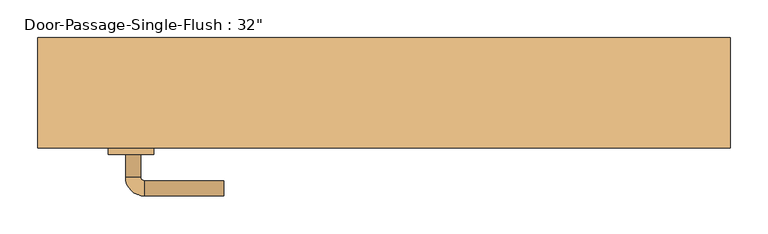
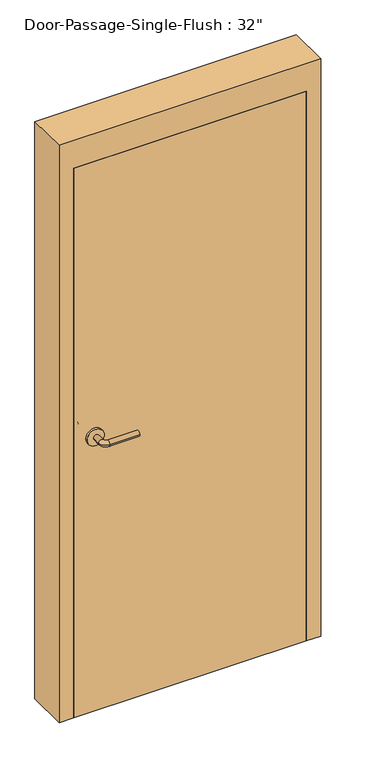
"""IFC4 building model written with IfcOpenShell, lengths in millimetres: door geometry."""

from ifc_helpers import new_model, si_unit, point, frame, frame_2d, origin, origin_with_axes, place, context, project, spatial, polyline, circle_curve, ellipse_curve, trimmed, segment, composite_curve, outline, extrude, faceted_brep, source, transform, mapped, element, save
from ifc_brep_helpers import plane_surface, cylinder_surface, revolved_surface, advanced_brep


def door_48051af7(model_context):
    return source(origin(), model_context, "Body", "SolidModel", [
        advanced_brep(
        [(-341.390625, 3.2375, 1016.0), (-321.390625, 3.2375, 1016.0), (-341.390625, 33.2375, 1016.0), (-321.390625, 33.2375, 1016.0), (-316.390625, 38.2375, 1016.0), (-316.390625, 58.2375, 1016.0), (-211.390625, 58.2375, 1016.0), (-211.390625, 38.2375, 1016.0)],
        [
            (0, 1, circle_curve(frame((-331.390625, 3.2375, 1016.0), z_axis=(0.0, -1.0, 0.0), x_axis=(1.0, 0.0, 0.0)), 10.0)),
            (1, 0, circle_curve(frame((-331.390625, 3.2375, 1016.0), z_axis=(0.0, -1.0, 0.0), x_axis=(1.0, 0.0, 0.0)), 10.0)),
            (0, 2),
            (2, 3, circle_curve(frame((-331.390625, 33.2375, 1016.0), z_axis=(0.0, -1.0, 0.0), x_axis=(1.0, 0.0, 0.0)), 10.0)),
            (3, 1),
            (3, 2, circle_curve(frame((-331.390625, 33.2375, 1016.0), z_axis=(0.0, -1.0, 0.0), x_axis=(1.0, 0.0, 0.0)), 10.0)),
            (4, 3, circle_curve(frame((-316.390625, 33.2375, 1016.0), z_axis=(0.0, 0.0, 1.0), x_axis=(-1.0, 0.0, 0.0)), 5.0)),
            (2, 5, circle_curve(frame((-316.390625, 33.2375, 1016.0), z_axis=(0.0, 0.0, -1.0), x_axis=(-1.0, 0.0, 0.0)), 25.0)),
            (5, 4, circle_curve(frame((-316.390625, 48.2375, 1016.0), z_axis=(-1.0, 0.0, 0.0), x_axis=(0.0, -1.0, 0.0)), 10.0)),
            (4, 5, circle_curve(frame((-316.390625, 48.2375, 1016.0), z_axis=(-1.0, 0.0, 0.0), x_axis=(0.0, -1.0, 0.0)), 10.0)),
            (6, 7, circle_curve(frame((-211.390625, 48.2375, 1016.0), z_axis=(1.0, 0.0, 0.0), x_axis=(0.0, -1.0, 0.0)), 10.0)),
            (7, 6, circle_curve(frame((-211.390625, 48.2375, 1016.0), z_axis=(1.0, 0.0, 0.0), x_axis=(0.0, -1.0, 0.0)), 10.0)),
            (5, 6),
            (7, 4),
        ],
        [
            plane_surface(frame((-331.390625, 3.2375, 1016.0), z_axis=(0.0, -1.0, 0.0), x_axis=(0.0, 0.0, 1.0))),
            cylinder_surface(frame((-331.390625, 3.2375, 1016.0), z_axis=(0.0, -1.0, 0.0), x_axis=(1.0, 0.0, 0.0)), 10.0),
            revolved_surface(trimmed(ellipse_curve(frame((-331.390625, 33.2375, 1016.0), z_axis=(0.0, -1.0, 0.0), x_axis=(1.0, 0.0, 0.0)), 10.0, 10.0), [point((-341.390625, 33.2375, 1016.0))], [point((-321.390625, 33.2375, 1016.0))], True, "CARTESIAN"), (-316.390625, 33.2375, 1016.0), (0.0, 0.0, -1.0)),
            revolved_surface(trimmed(ellipse_curve(frame((-331.390625, 33.2375, 1016.0), z_axis=(0.0, -1.0, 0.0), x_axis=(1.0, 0.0, 0.0)), 10.0, 10.0), [point((-321.390625, 33.2375, 1016.0))], [point((-341.390625, 33.2375, 1016.0))], True, "CARTESIAN"), (-316.390625, 33.2375, 1016.0), (0.0, 0.0, -1.0)),
            plane_surface(frame((-211.390625, 48.2375, 1016.0), z_axis=(1.0, 0.0, 0.0), x_axis=(0.0, 0.0, 1.0))),
            cylinder_surface(frame((-316.390625, 48.2375, 1016.0), z_axis=(-1.0, 0.0, 0.0), x_axis=(0.0, -1.0, 0.0)), 10.0),
        ],
        [
            (0, [[1, 2]]),
            (1, [[-1, 3, 4, 5]]),
            (1, [[-2, -5, 6, -3]]),
            (2, [[7, -4, 8, 9]]),
            (3, [[-8, -6, -7, 10]]),
            (4, [[11, 12]]),
            (5, [[-9, 13, -12, 14]]),
            (5, [[-10, -14, -11, -13]]),
        ],
    ),
        extrude(outline(composite_curve([segment(trimmed(circle_curve(frame_2d((1016.0, -333.890625)), 30.0), [point((1016.0, -363.890625))], [point((1016.0, -303.890625))], False, "CARTESIAN"), True, "CONTINUOUS"), segment(trimmed(circle_curve(frame_2d((1016.0, -333.890625)), 30.0), [point((1016.0, -303.890625))], [point((1016.0, -363.890625))], False, "CARTESIAN"), True, "CONTINUOUS")], self_intersect=False)), frame((0.0, -4.7625, 0.0), z_axis=(0.0, 1.0, 0.0), x_axis=(0.0, 0.0, 1.0)), (0.0, 0.0, 1.0), 8.0),
        advanced_brep(
        [(-341.390625, -57.2125, 1016.0), (-321.390625, -57.2125, 1016.0), (-321.390625, -87.2125, 1016.0), (-341.390625, -87.2125, 1016.0), (-316.390625, -92.2125, 1016.0), (-316.390625, -112.2125, 1016.0), (-211.390625, -112.2125, 1016.0), (-211.390625, -92.2125, 1016.0)],
        [
            (0, 1, circle_curve(frame((-331.390625, -57.2125, 1016.0), z_axis=(0.0, 1.0, 0.0), x_axis=(1.0, 0.0, 0.0)), 10.0)),
            (1, 0, circle_curve(frame((-331.390625, -57.2125, 1016.0), z_axis=(0.0, 1.0, 0.0), x_axis=(1.0, 0.0, 0.0)), 10.0)),
            (1, 2),
            (2, 3, circle_curve(frame((-331.390625, -87.2125, 1016.0), z_axis=(0.0, 1.0, 0.0), x_axis=(1.0, 0.0, 0.0)), 10.0)),
            (3, 0),
            (3, 2, circle_curve(frame((-331.390625, -87.2125, 1016.0), z_axis=(0.0, 1.0, 0.0), x_axis=(1.0, 0.0, 0.0)), 10.0)),
            (4, 5, circle_curve(frame((-316.390625, -102.2125, 1016.0), z_axis=(-1.0, 0.0, 0.0), x_axis=(0.0, 1.0, 0.0)), 10.0)),
            (5, 3, circle_curve(frame((-316.390625, -87.2125, 1016.0), z_axis=(0.0, 0.0, -1.0), x_axis=(-1.0, 0.0, 0.0)), 25.0)),
            (2, 4, circle_curve(frame((-316.390625, -87.2125, 1016.0), z_axis=(0.0, 0.0, 1.0), x_axis=(-1.0, 0.0, 0.0)), 5.0)),
            (5, 4, circle_curve(frame((-316.390625, -102.2125, 1016.0), z_axis=(-1.0, 0.0, 0.0), x_axis=(0.0, 1.0, 0.0)), 10.0)),
            (6, 7, circle_curve(frame((-211.390625, -102.2125, 1016.0), z_axis=(1.0, 0.0, 0.0), x_axis=(0.0, 1.0, 0.0)), 10.0)),
            (7, 6, circle_curve(frame((-211.390625, -102.2125, 1016.0), z_axis=(1.0, 0.0, 0.0), x_axis=(0.0, 1.0, 0.0)), 10.0)),
            (4, 7),
            (6, 5),
        ],
        [
            plane_surface(frame((-331.390625, -57.2125, 1016.0), z_axis=(0.0, 1.0, 0.0), x_axis=(0.0, 0.0, 1.0))),
            cylinder_surface(frame((-331.390625, -57.2125, 1016.0), z_axis=(0.0, 1.0, 0.0), x_axis=(1.0, 0.0, 0.0)), 10.0),
            revolved_surface(trimmed(ellipse_curve(frame((-331.390625, -87.2125, 1016.0), z_axis=(0.0, -1.0, 0.0), x_axis=(1.0, 0.0, 0.0)), 10.0, 10.0), [point((-341.390625, -87.2125, 1016.0))], [point((-321.390625, -87.2125, 1016.0))], True, "CARTESIAN"), (-316.390625, -87.2125, 1016.0), (0.0, 0.0, -1.0)),
            revolved_surface(trimmed(ellipse_curve(frame((-331.390625, -87.2125, 1016.0), z_axis=(0.0, -1.0, 0.0), x_axis=(1.0, 0.0, 0.0)), 10.0, 10.0), [point((-321.390625, -87.2125, 1016.0))], [point((-341.390625, -87.2125, 1016.0))], True, "CARTESIAN"), (-316.390625, -87.2125, 1016.0), (0.0, 0.0, -1.0)),
            plane_surface(frame((-211.390625, -102.2125, 1016.0), z_axis=(1.0, 0.0, 0.0), x_axis=(0.0, 0.0, 1.0))),
            cylinder_surface(frame((-316.390625, -102.2125, 1016.0), z_axis=(-1.0, 0.0, 0.0), x_axis=(0.0, 1.0, 0.0)), 10.0),
        ],
        [
            (0, [[1, 2]]),
            (1, [[3, 4, 5, -2]]),
            (1, [[-5, 6, -3, -1]]),
            (2, [[7, 8, -4, 9]]),
            (3, [[10, -9, -6, -8]]),
            (4, [[11, 12]]),
            (5, [[13, -11, 14, -7]]),
            (5, [[-14, -12, -13, -10]]),
        ],
    ),
        extrude(outline(composite_curve([segment(trimmed(circle_curve(frame_2d((1016.0, -333.890625)), 30.0), [point((1016.0, -363.890625))], [point((1016.0, -303.890625))], False, "CARTESIAN"), True, "CONTINUOUS"), segment(trimmed(circle_curve(frame_2d((1016.0, -333.890625)), 30.0), [point((1016.0, -303.890625))], [point((1016.0, -363.890625))], False, "CARTESIAN"), True, "CONTINUOUS")], self_intersect=False)), frame((0.0, -57.2125, 0.0), z_axis=(0.0, 1.0, 0.0), x_axis=(0.0, 0.0, 1.0)), (0.0, 0.0, 1.0), 8.0),
        faceted_brep([(406.4, 0.0, 0.0), (390.525, 0.0, 0.0), (390.525, 47.625, 0.0), (406.4, 47.625, 0.0), (406.4, 96.8375, 0.0), (457.2, 96.8375, 0.0), (457.2, -49.2125, 0.0), (406.4, -49.2125, 0.0), (406.4, -49.2125, 2032.0), (406.4, 0.0, 2032.0), (457.2, -49.2125, 2133.6), (-457.2, -49.2125, 2133.6), (-457.2, -49.2125, 0.0), (-406.4, -49.2125, 0.0), (-406.4, -49.2125, 2032.0), (457.2, 96.8375, 2133.6), (406.4, 96.8375, 2032.0), (-406.4, 96.8375, 2032.0), (-406.4, 96.8375, 0.0), (-457.2, 96.8375, 0.0), (-457.2, 96.8375, 2133.6), (406.4, 47.625, 2032.0), (390.525, 47.625, 2016.125), (-390.525, 47.625, 2016.125), (-390.525, 47.625, 0.0), (-406.4, 47.625, 0.0), (-406.4, 47.625, 2032.0), (390.525, 0.0, 2016.125), (-406.4, 0.0, 2032.0), (-406.4, 0.0, 0.0), (-390.525, 0.0, 0.0), (-390.525, 0.0, 2016.125)], [[[0, 1, 2, 3, 4, 5, 6, 7]], [[7, 8, 9, 0]], [[6, 10, 11, 12, 13, 14, 8, 7]], [[5, 15, 10, 6]], [[4, 16, 17, 18, 19, 20, 15, 5]], [[3, 21, 16, 4]], [[2, 22, 23, 24, 25, 26, 21, 3]], [[1, 27, 22, 2]], [[0, 9, 28, 29, 30, 31, 27, 1]], [[8, 14, 28, 9]], [[16, 21, 26, 17]], [[22, 27, 31, 23]], [[12, 19, 18, 25, 24, 30, 29, 13]], [[13, 29, 28, 14]], [[11, 20, 19, 12]], [[17, 26, 25, 18]], [[23, 31, 30, 24]], [[15, 20, 11, 10]]]),
        extrude(outline(polyline([(406.4, -4.7625), (406.4, -49.2125), (-406.4, -49.2125), (-406.4, -4.7625), (406.4, -4.7625)])), origin_with_axes(), (0.0, 0.0, 1.0), 2032.0),
    ])


if __name__ == "__main__":
    model = new_model("IFC4")
    model_context = context("Model", 3, world=origin())
    ifc_project = project(units=[si_unit("LENGTHUNIT", "METRE", prefix="MILLI")], contexts=[model_context])
    site = spatial("IfcSite", under=ifc_project)
    building = spatial("IfcBuilding", under=site)
    placement = place(None, origin())
    door_shape = door_48051af7(model_context)
    element("IfcDoor", 1, ObjectType="Door-Passage-Single-Flush : 32\"", at=placement, inside=building, context=model_context, shape_type="MappedRepresentation", body=[
        mapped(door_shape, transform((0.0, 0.0, 0.0), x_axis=(1.0, 0.0, 0.0), y_axis=(0.0, 1.0, 0.0), z_axis=(0.0, 0.0, 1.0))),
    ])
    save(model, "model.ifc")

# Revit data of these elements
# Type "Door-Passage-Single-Flush : 32\""
#   Type Mark = "42"
#   Assembly Code = "B2030200"
#   Analytic Construction = "Wooden"
#   Thickness = 0' - 1 3/4"
#   Thermal Resistance (R) = 0.455703 (m²·K)/W
#   Swing Angle [instance default] = 90.00°
#   Strike Height = 3' - 4"
#   Rough Width [instance default] = 3' - 0"
#   Rough Height [instance default] = 7' - 0"
#   MF Opening Height [instance default] = 0' - 4"
#   MF Opening Width [instance default] = 0' - 4"
#   Inset Calculate [instance default] = 0' - 4"
#   Masonry Inset [instance default] = 0' - 1"
#   Height = 6' - 8"
#   Width = 2' - 8"
#   Heat Transfer Coefficient (U) = 2.19465 W/(m²·K)
#   Masonry Frame Depth = 0' - 5 3/4"
#   Masonry Frame [instance default] = yes
#   Function = 1
#   Dry Wall Frame [instance default] = no
#   Panel Material = Wood - Birch
#   Frame Material = Metal - Paint Finish - Grey
#   Door Handle Material = Aluminum
#   Visual Light Transmittance = 0
#   Solar Heat Gain Coefficient = 0
#   Wall Closure = (empty or 0)
# Element 1 (IfcDoor, "Door-Passage-Single-Flush : 32\"")
#   Materials on its faces: "Aluminum", "Metal - Paint Finish - Grey", "Wood - Birch"
# Materials
#   "Wood - Birch": class "Wood", colour RGB 166 116 52, transparency 0, Cost = 0
#   "Metal - Paint Finish - Grey": class "Paint", colour RGB 104 104 104, transparency 0, Cost = 0
#   "Aluminum": class "Metal", colour RGB 247 247 247, transparency 0, Description = "Aluminum 6061", Cost = 0
